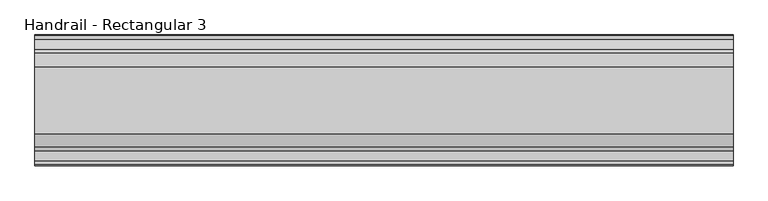
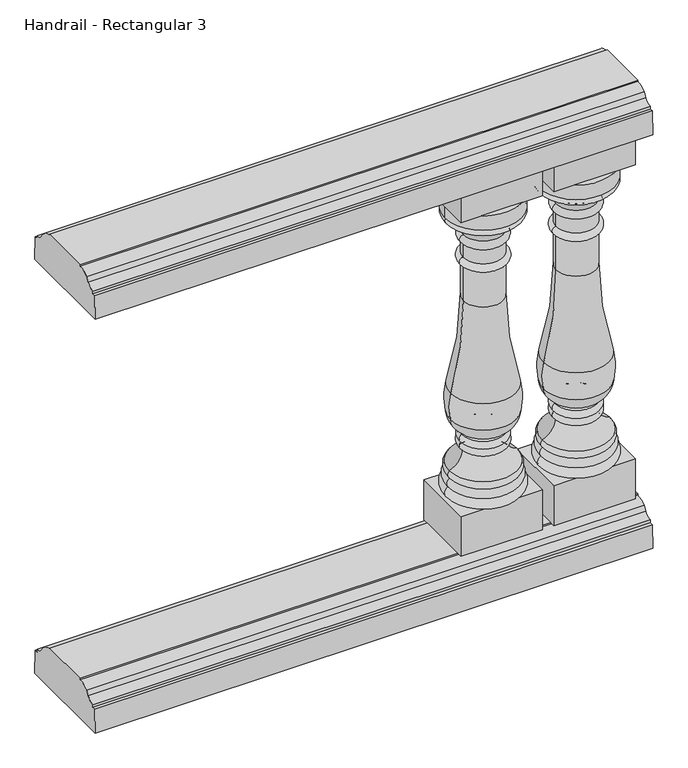
"""IFC4 building model written with IfcOpenShell, lengths in millimetres: railing geometry, Handrail - Rectangular 3."""

from ifc_helpers import new_model, si_unit, point, frame, frame_2d, origin, place, context, project, spatial, polyline, circle_curve, ellipse_curve, trimmed, segment, composite_curve, outline, extrude, source, transform, mapped, element, save
from ifc_brep_helpers import plane_surface, cylinder_surface, revolved_surface, advanced_brep


def handrail_rectangular_3_6dd137a3(model_context):
    return source(origin(), model_context, "Body", "SolidModel", [
        extrude(outline(composite_curve([segment(trimmed(circle_curve(frame_2d((-1771.1852268, 1054.89375)), 19.84375), [point((-1771.1852268, 1035.05))], [point((-1754.064785, 1044.8605607))], True, "CARTESIAN"), True, "CONTINUOUS"), segment(polyline([(-1754.064785, 1044.8605607), (-1747.604713, 1054.3201059)]), True, "CONTINUOUS"), segment(trimmed(circle_curve(frame_2d((-1723.5602268, 1027.90625)), 35.71875), [point((-1747.604713, 1054.3201059))], [point((-1723.5602268, 1063.625))], False, "CARTESIAN"), True, "CONTINUOUS"), segment(polyline([(-1723.5602268, 1063.625), (-1723.5602268, 1066.8), (-1607.6727268, 1066.8), (-1607.6727268, 1063.625)]), True, "CONTINUOUS"), segment(trimmed(circle_curve(frame_2d((-1607.6727268, 1027.90625)), 35.71875), [point((-1607.6727268, 1063.625))], [point((-1583.6282406, 1054.3201059))], False, "CARTESIAN"), True, "CONTINUOUS"), segment(polyline([(-1583.6282406, 1054.3201059), (-1577.1681686, 1044.8605607)]), True, "CONTINUOUS"), segment(trimmed(circle_curve(frame_2d((-1560.0477268, 1054.89375)), 19.84375), [point((-1577.1681686, 1044.8605607))], [point((-1560.0477268, 1035.05))], True, "CARTESIAN"), True, "CONTINUOUS"), segment(polyline([(-1560.0477268, 1035.05), (-1560.0477268, 1028.7), (-1552.9039768, 1028.7), (-1551.3164768, 974.725), (-1779.9164768, 974.725), (-1778.3289768, 1028.7), (-1771.1852268, 1028.7), (-1771.1852268, 1035.05)]), True, "CONTINUOUS")], self_intersect=False)), frame((11389.2521895, 0.0, 0.0), z_axis=(1.0, 0.0, 0.0), x_axis=(0.0, 1.0, 0.0)), (0.0, 0.0, 1.0), 1219.2),
        extrude(outline(composite_curve([segment(trimmed(circle_curve(frame_2d((-1771.1852268, 99.21875)), 19.84375), [point((-1771.1852268, 79.375))], [point((-1754.064785, 89.1855607))], True, "CARTESIAN"), True, "CONTINUOUS"), segment(polyline([(-1754.064785, 89.1855607), (-1747.604713, 98.6451059)]), True, "CONTINUOUS"), segment(trimmed(circle_curve(frame_2d((-1723.5602268, 72.23125)), 35.71875), [point((-1747.604713, 98.6451059))], [point((-1723.5602268, 107.95))], False, "CARTESIAN"), True, "CONTINUOUS"), segment(polyline([(-1723.5602268, 107.95), (-1723.5602268, 111.125), (-1607.6727268, 111.125), (-1607.6727268, 107.95)]), True, "CONTINUOUS"), segment(trimmed(circle_curve(frame_2d((-1607.6727268, 72.23125)), 35.71875), [point((-1607.6727268, 107.95))], [point((-1583.6282406, 98.6451059))], False, "CARTESIAN"), True, "CONTINUOUS"), segment(polyline([(-1583.6282406, 98.6451059), (-1577.1681686, 89.1855607)]), True, "CONTINUOUS"), segment(trimmed(circle_curve(frame_2d((-1560.0477268, 99.21875)), 19.84375), [point((-1577.1681686, 89.1855607))], [point((-1560.0477268, 79.375))], True, "CARTESIAN"), True, "CONTINUOUS"), segment(polyline([(-1560.0477268, 79.375), (-1560.0477268, 73.025), (-1552.9039768, 73.025), (-1551.3164768, 19.05), (-1779.9164768, 19.05), (-1778.3289768, 73.025), (-1771.1852268, 73.025), (-1771.1852268, 79.375)]), True, "CONTINUOUS")], self_intersect=False)), frame((11389.2521895, 0.0, 0.0), z_axis=(1.0, 0.0, 0.0), x_axis=(0.0, 1.0, 0.0)), (0.0, 0.0, 1.0), 1219.2),
        advanced_brep(
        [(12423.5084395, -1665.6164768, 849.3125), (12590.1959395, -1665.6164768, 849.3125), (12590.1959395, -1665.6164768, 882.65), (12423.5084395, -1665.6164768, 882.65), (12426.6834395, -1665.6164768, 849.3125), (12587.0209395, -1665.6164768, 849.3125), (12426.6834395, -1665.6164768, 835.025), (12587.0209395, -1665.6164768, 835.025), (12463.1959395, -1665.6164768, 796.925), (12550.5084395, -1665.6164768, 796.925), (12463.1959395, -1665.6164768, 777.875), (12550.5084395, -1665.6164768, 777.875), (12463.1959395, -1665.6164768, 744.5375), (12550.5084395, -1665.6164768, 744.5375), (12463.1959395, -1665.6164768, 727.075), (12550.5084395, -1665.6164768, 727.075), (12463.1959395, -1665.6164768, 644.525), (12550.5084395, -1665.6164768, 644.525), (12436.0074221, -1665.6164768, 440.2065586), (12577.696957, -1665.6164768, 440.2065586), (12434.8170661, -1665.6164768, 379.6643134), (12578.887313, -1665.6164768, 379.6643134), (12462.0281246, -1665.6164768, 340.8286685), (12551.6762545, -1665.6164768, 340.8286685), (12460.3028429, -1665.6164768, 336.3463085), (12553.4015362, -1665.6164768, 336.3463085), (12459.2271895, -1665.6164768, 319.0875), (12554.4771895, -1665.6164768, 319.0875), (12462.4021895, -1665.6164768, 301.625), (12551.3021895, -1665.6164768, 301.625), (12433.0334395, -1665.6164768, 261.9375), (12580.6709395, -1665.6164768, 261.9375), (12433.8271895, -1665.6164768, 244.475), (12579.8771895, -1665.6164768, 244.475), (12429.8584395, -1665.6164768, 225.425), (12583.8459395, -1665.6164768, 225.425), (12426.6834395, -1665.6164768, 203.2), (12587.0209395, -1665.6164768, 203.2), (12506.8521895, -1665.6164768, 203.2), (12506.8521895, -1665.6164768, 882.65)],
        [
            (0, 1, circle_curve(frame((12506.8521895, -1665.6164768, 849.3125), z_axis=(0.0, 0.0, 1.0), x_axis=(1.0, 0.0, 0.0)), 83.34375)),
            (1, 2),
            (2, 3, circle_curve(frame((12506.8521895, -1665.6164768, 882.65), z_axis=(0.0, 0.0, -1.0), x_axis=(1.0, 0.0, 0.0)), 83.34375)),
            (3, 0),
            (1, 0, circle_curve(frame((12506.8521895, -1665.6164768, 849.3125), z_axis=(0.0, 0.0, 1.0), x_axis=(1.0, 0.0, 0.0)), 83.34375)),
            (3, 2, circle_curve(frame((12506.8521895, -1665.6164768, 882.65), z_axis=(0.0, 0.0, -1.0), x_axis=(1.0, 0.0, 0.0)), 83.34375)),
            (4, 5, circle_curve(frame((12506.8521895, -1665.6164768, 849.3125), z_axis=(0.0, 0.0, 1.0), x_axis=(1.0, 0.0, 0.0)), 80.16875)),
            (5, 1),
            (0, 4),
            (5, 4, circle_curve(frame((12506.8521895, -1665.6164768, 849.3125), z_axis=(0.0, 0.0, 1.0), x_axis=(1.0, 0.0, 0.0)), 80.16875)),
            (6, 7, circle_curve(frame((12506.8521895, -1665.6164768, 835.025), z_axis=(0.0, 0.0, 1.0), x_axis=(1.0, 0.0, 0.0)), 80.16875)),
            (7, 5, circle_curve(frame((12580.5717208, -1665.6164768, 842.16875), z_axis=(0.0, -1.0, 0.0), x_axis=(1.0, 0.0, 0.0)), 9.6242187)),
            (4, 6, circle_curve(frame((12433.1326583, -1665.6164768, 842.16875), z_axis=(0.0, -1.0, 0.0), x_axis=(-1.0, 0.0, 0.0)), 9.6242187)),
            (7, 6, circle_curve(frame((12506.8521895, -1665.6164768, 835.025), z_axis=(0.0, 0.0, 1.0), x_axis=(1.0, 0.0, 0.0)), 80.16875)),
            (8, 9, circle_curve(frame((12506.8521895, -1665.6164768, 796.925), z_axis=(0.0, 0.0, 1.0), x_axis=(1.0, 0.0, 0.0)), 43.65625)),
            (9, 7, circle_curve(frame((12605.925244, -1665.6164768, 780.362802), z_axis=(0.0, 1.0, 0.0), x_axis=(1.0, 0.0, 0.0)), 57.8388159)),
            (6, 8, circle_curve(frame((12407.7791351, -1665.6164768, 780.362802), z_axis=(0.0, 1.0, 0.0), x_axis=(-1.0, 0.0, 0.0)), 57.8388159)),
            (9, 8, circle_curve(frame((12506.8521895, -1665.6164768, 796.925), z_axis=(0.0, 0.0, 1.0), x_axis=(1.0, 0.0, 0.0)), 43.65625)),
            (10, 11, circle_curve(frame((12506.8521895, -1665.6164768, 777.875), z_axis=(0.0, 0.0, 1.0), x_axis=(1.0, 0.0, 0.0)), 43.65625)),
            (11, 9, circle_curve(frame((12548.7621895, -1665.6164768, 787.4), z_axis=(0.0, -1.0, 0.0), x_axis=(1.0, 0.0, 0.0)), 9.68375)),
            (8, 10, circle_curve(frame((12464.9421895, -1665.6164768, 787.4), z_axis=(0.0, -1.0, 0.0), x_axis=(-1.0, 0.0, 0.0)), 9.68375)),
            (11, 10, circle_curve(frame((12506.8521895, -1665.6164768, 777.875), z_axis=(0.0, 0.0, 1.0), x_axis=(1.0, 0.0, 0.0)), 43.65625)),
            (12, 13, circle_curve(frame((12506.8521895, -1665.6164768, 744.5375), z_axis=(0.0, 0.0, 1.0), x_axis=(1.0, 0.0, 0.0)), 43.65625)),
            (13, 11),
            (10, 12),
            (13, 12, circle_curve(frame((12506.8521895, -1665.6164768, 744.5375), z_axis=(0.0, 0.0, 1.0), x_axis=(1.0, 0.0, 0.0)), 43.65625)),
            (14, 15, circle_curve(frame((12506.8521895, -1665.6164768, 727.075), z_axis=(0.0, 0.0, 1.0), x_axis=(1.0, 0.0, 0.0)), 43.65625)),
            (15, 13, circle_curve(frame((12550.5084395, -1665.6164768, 735.80625), z_axis=(0.0, -1.0, 0.0), x_axis=(1.0, 0.0, 0.0)), 8.73125)),
            (12, 14, circle_curve(frame((12463.1959395, -1665.6164768, 735.80625), z_axis=(0.0, -1.0, 0.0), x_axis=(-1.0, 0.0, 0.0)), 8.73125)),
            (15, 14, circle_curve(frame((12506.8521895, -1665.6164768, 727.075), z_axis=(0.0, 0.0, 1.0), x_axis=(1.0, 0.0, 0.0)), 43.65625)),
            (16, 17, circle_curve(frame((12506.8521895, -1665.6164768, 644.525), z_axis=(0.0, 0.0, 1.0), x_axis=(1.0, 0.0, 0.0)), 43.65625)),
            (17, 15),
            (14, 16),
            (17, 16, circle_curve(frame((12506.8521895, -1665.6164768, 644.525), z_axis=(0.0, 0.0, 1.0), x_axis=(1.0, 0.0, 0.0)), 43.65625)),
            (18, 19, circle_curve(frame((12506.8521895, -1665.6164768, 440.2065586), z_axis=(0.0, 0.0, 1.0), x_axis=(1.0, 0.0, 0.0)), 70.8447675)),
            (19, 17, circle_curve(frame((13285.2851891, -1665.6164768, 638.333048), z_axis=(0.0, 1.0, 0.0), x_axis=(1.0, 0.0, 0.0)), 734.8028389)),
            (16, 18, circle_curve(frame((11728.41919, -1665.6164768, 638.333048), z_axis=(0.0, 1.0, 0.0), x_axis=(-1.0, 0.0, 0.0)), 734.8028389)),
            (19, 18, circle_curve(frame((12506.8521895, -1665.6164768, 440.2065586), z_axis=(0.0, 0.0, 1.0), x_axis=(1.0, 0.0, 0.0)), 70.8447675)),
            (20, 21, circle_curve(frame((12506.8521895, -1665.6164768, 379.6643134), z_axis=(0.0, 0.0, 1.0), x_axis=(1.0, 0.0, 0.0)), 72.0351235)),
            (21, 19, circle_curve(frame((12419.7983349, -1665.6164768, 406.819198), z_axis=(0.0, -1.0, 0.0), x_axis=(1.0, 0.0, 0.0)), 161.3898718)),
            (18, 20, circle_curve(frame((12593.9060442, -1665.6164768, 406.819198), z_axis=(0.0, -1.0, 0.0), x_axis=(-1.0, 0.0, 0.0)), 161.3898718)),
            (21, 20, circle_curve(frame((12506.8521895, -1665.6164768, 379.6643134), z_axis=(0.0, 0.0, 1.0), x_axis=(1.0, 0.0, 0.0)), 72.0351235)),
            (22, 23, circle_curve(frame((12506.8521895, -1665.6164768, 340.8286685), z_axis=(0.0, 0.0, 1.0), x_axis=(1.0, 0.0, 0.0)), 44.8240649)),
            (23, 21, circle_curve(frame((12529.1572912, -1665.6164768, 385.5579203), z_axis=(0.0, -1.0, 0.0), x_axis=(1.0, 0.0, 0.0)), 50.0780358)),
            (20, 22, circle_curve(frame((12484.5470879, -1665.6164768, 385.5579203), z_axis=(0.0, -1.0, 0.0), x_axis=(-1.0, 0.0, 0.0)), 50.0780358)),
            (23, 22, circle_curve(frame((12506.8521895, -1665.6164768, 340.8286685), z_axis=(0.0, 0.0, 1.0), x_axis=(1.0, 0.0, 0.0)), 44.8240649)),
            (24, 25, circle_curve(frame((12506.8521895, -1665.6164768, 336.3463085), z_axis=(0.0, 0.0, 1.0), x_axis=(1.0, 0.0, 0.0)), 46.5493467)),
            (25, 23, circle_curve(frame((12554.4771895, -1665.6164768, 339.3335472), z_axis=(0.0, 1.0, 0.0), x_axis=(1.0, 0.0, 0.0)), 3.175)),
            (22, 24, circle_curve(frame((12459.2271895, -1665.6164768, 339.3335472), z_axis=(0.0, 1.0, 0.0), x_axis=(-1.0, 0.0, 0.0)), 3.175)),
            (25, 24, circle_curve(frame((12506.8521895, -1665.6164768, 336.3463085), z_axis=(0.0, 0.0, 1.0), x_axis=(1.0, 0.0, 0.0)), 46.5493467)),
            (26, 27, circle_curve(frame((12506.8521895, -1665.6164768, 319.0875), z_axis=(0.0, 0.0, 1.0), x_axis=(1.0, 0.0, 0.0)), 47.625)),
            (27, 25, circle_curve(frame((12549.4008248, -1665.6164768, 327.4340404), z_axis=(0.0, -1.0, 0.0), x_axis=(1.0, 0.0, 0.0)), 9.7690437)),
            (24, 26, circle_curve(frame((12464.3035543, -1665.6164768, 327.4340404), z_axis=(0.0, -1.0, 0.0), x_axis=(-1.0, 0.0, 0.0)), 9.7690437)),
            (27, 26, circle_curve(frame((12506.8521895, -1665.6164768, 319.0875), z_axis=(0.0, 0.0, 1.0), x_axis=(1.0, 0.0, 0.0)), 47.625)),
            (28, 29, circle_curve(frame((12506.8521895, -1665.6164768, 301.625), z_axis=(0.0, 0.0, 1.0), x_axis=(1.0, 0.0, 0.0)), 44.45)),
            (29, 27, circle_curve(frame((12549.8635177, -1665.6164768, 310.9064631), z_axis=(0.0, -1.0, 0.0), x_axis=(1.0, 0.0, 0.0)), 9.3923018)),
            (26, 28, circle_curve(frame((12463.8408614, -1665.6164768, 310.9064631), z_axis=(0.0, -1.0, 0.0), x_axis=(-1.0, 0.0, 0.0)), 9.3923018)),
            (29, 28, circle_curve(frame((12506.8521895, -1665.6164768, 301.625), z_axis=(0.0, 0.0, 1.0), x_axis=(1.0, 0.0, 0.0)), 44.45)),
            (30, 31, circle_curve(frame((12506.8521895, -1665.6164768, 261.9375), z_axis=(0.0, 0.0, 1.0), x_axis=(1.0, 0.0, 0.0)), 73.81875)),
            (31, 29, circle_curve(frame((12592.8024429, -1665.6164768, 301.625), z_axis=(0.0, 1.0, 0.0), x_axis=(1.0, 0.0, 0.0)), 41.5002534)),
            (28, 30, circle_curve(frame((12420.9019362, -1665.6164768, 301.625), z_axis=(0.0, 1.0, 0.0), x_axis=(-1.0, 0.0, 0.0)), 41.5002534)),
            (31, 30, circle_curve(frame((12506.8521895, -1665.6164768, 261.9375), z_axis=(0.0, 0.0, 1.0), x_axis=(1.0, 0.0, 0.0)), 73.81875)),
            (32, 33, circle_curve(frame((12506.8521895, -1665.6164768, 244.475), z_axis=(0.0, 0.0, 1.0), x_axis=(1.0, 0.0, 0.0)), 73.025)),
            (33, 31, circle_curve(frame((12571.3664257, -1665.6164768, 253.6111427), z_axis=(0.0, -1.0, 0.0), x_axis=(1.0, 0.0, 0.0)), 12.4860804)),
            (30, 32, circle_curve(frame((12442.3379534, -1665.6164768, 253.6111427), z_axis=(0.0, -1.0, 0.0), x_axis=(-1.0, 0.0, 0.0)), 12.4860804)),
            (33, 32, circle_curve(frame((12506.8521895, -1665.6164768, 244.475), z_axis=(0.0, 0.0, 1.0), x_axis=(1.0, 0.0, 0.0)), 73.025)),
            (34, 35, circle_curve(frame((12506.8521895, -1665.6164768, 225.425), z_axis=(0.0, 0.0, 1.0), x_axis=(1.0, 0.0, 0.0)), 76.99375)),
            (35, 33, circle_curve(frame((12573.2024736, -1665.6164768, 233.1460227), z_axis=(0.0, -1.0, 0.0), x_axis=(1.0, 0.0, 0.0)), 13.1490516)),
            (32, 34, circle_curve(frame((12440.5019054, -1665.6164768, 233.1460227), z_axis=(0.0, -1.0, 0.0), x_axis=(-1.0, 0.0, 0.0)), 13.1490516)),
            (35, 34, circle_curve(frame((12506.8521895, -1665.6164768, 225.425), z_axis=(0.0, 0.0, 1.0), x_axis=(1.0, 0.0, 0.0)), 76.99375)),
            (36, 37, circle_curve(frame((12506.8521895, -1665.6164768, 203.2), z_axis=(0.0, 0.0, 1.0), x_axis=(1.0, 0.0, 0.0)), 80.16875)),
            (37, 35, circle_curve(frame((12576.8722788, -1665.6164768, 213.089477), z_axis=(0.0, -1.0, 0.0), x_axis=(1.0, 0.0, 0.0)), 14.1702883)),
            (34, 36, circle_curve(frame((12436.8321003, -1665.6164768, 213.089477), z_axis=(0.0, -1.0, 0.0), x_axis=(-1.0, 0.0, 0.0)), 14.1702883)),
            (37, 36, circle_curve(frame((12506.8521895, -1665.6164768, 203.2), z_axis=(0.0, 0.0, 1.0), x_axis=(1.0, 0.0, 0.0)), 80.16875)),
            (38, 37),
            (36, 38),
            (2, 39),
            (39, 3),
        ],
        [
            cylinder_surface(frame((12506.8521895, -1665.6164768, 831.85), z_axis=(0.0, 0.0, -1.0), x_axis=(1.0, 0.0, 0.0)), 83.34375),
            plane_surface(frame((12506.8521895, -1665.6164768, 849.3125), z_axis=(0.0, 0.0, -1.0), x_axis=(1.0, 0.0, 0.0))),
            revolved_surface(trimmed(ellipse_curve(frame((12580.5717208, -1665.6164768, 842.16875), z_axis=(0.0, 1.0, 0.0), x_axis=(1.0, 0.0, 0.0)), 9.6242187, 9.6242187), [point((12587.0209395, -1665.6164768, 849.3125))], [point((12587.0209395, -1665.6164768, 835.025))], True, "CARTESIAN"), (12506.8521895, -1665.6164768, 831.85), (0.0, 0.0, -1.0)),
            revolved_surface(trimmed(ellipse_curve(frame((12605.925244, -1665.6164768, 780.362802), z_axis=(0.0, -1.0, 0.0), x_axis=(1.0, 0.0, 0.0)), 57.8388159, 57.8388159), [point((12587.0209395, -1665.6164768, 835.025))], [point((12550.5084395, -1665.6164768, 796.925))], True, "CARTESIAN"), (12506.8521895, -1665.6164768, 831.85), (0.0, 0.0, -1.0)),
            revolved_surface(trimmed(ellipse_curve(frame((12548.7621895, -1665.6164768, 787.4), z_axis=(0.0, 1.0, 0.0), x_axis=(1.0, 0.0, 0.0)), 9.68375, 9.68375), [point((12550.5084395, -1665.6164768, 796.925))], [point((12550.5084395, -1665.6164768, 777.875))], True, "CARTESIAN"), (12506.8521895, -1665.6164768, 831.85), (0.0, 0.0, -1.0)),
            cylinder_surface(frame((12506.8521895, -1665.6164768, 831.85), z_axis=(0.0, 0.0, -1.0), x_axis=(1.0, 0.0, 0.0)), 43.65625),
            revolved_surface(trimmed(ellipse_curve(frame((12550.5084395, -1665.6164768, 735.80625), z_axis=(0.0, 1.0, 0.0), x_axis=(1.0, 0.0, 0.0)), 8.73125, 8.73125), [point((12550.5084395, -1665.6164768, 744.5375))], [point((12550.5084395, -1665.6164768, 727.075))], True, "CARTESIAN"), (12506.8521895, -1665.6164768, 831.85), (0.0, 0.0, -1.0)),
            revolved_surface(trimmed(ellipse_curve(frame((13285.2851891, -1665.6164768, 638.333048), z_axis=(0.0, -1.0, 0.0), x_axis=(1.0, 0.0, 0.0)), 734.8028389, 734.8028389), [point((12550.5084395, -1665.6164768, 644.525))], [point((12577.696957, -1665.6164768, 440.2065586))], True, "CARTESIAN"), (12506.8521895, -1665.6164768, 831.85), (0.0, 0.0, -1.0)),
            revolved_surface(trimmed(ellipse_curve(frame((12419.7983349, -1665.6164768, 406.819198), z_axis=(0.0, 1.0, 0.0), x_axis=(1.0, 0.0, 0.0)), 161.3898718, 161.3898718), [point((12577.696957, -1665.6164768, 440.2065586))], [point((12578.887313, -1665.6164768, 379.6643134))], True, "CARTESIAN"), (12506.8521895, -1665.6164768, 831.85), (0.0, 0.0, -1.0)),
            revolved_surface(trimmed(ellipse_curve(frame((12529.1572912, -1665.6164768, 385.5579203), z_axis=(0.0, 1.0, 0.0), x_axis=(1.0, 0.0, 0.0)), 50.0780358, 50.0780358), [point((12578.887313, -1665.6164768, 379.6643134))], [point((12551.6762545, -1665.6164768, 340.8286685))], True, "CARTESIAN"), (12506.8521895, -1665.6164768, 831.85), (0.0, 0.0, -1.0)),
            revolved_surface(trimmed(ellipse_curve(frame((12554.4771895, -1665.6164768, 339.3335472), z_axis=(0.0, -1.0, 0.0), x_axis=(1.0, 0.0, 0.0)), 3.175, 3.175), [point((12551.6762545, -1665.6164768, 340.8286685))], [point((12553.4015362, -1665.6164768, 336.3463085))], True, "CARTESIAN"), (12506.8521895, -1665.6164768, 831.85), (0.0, 0.0, -1.0)),
            revolved_surface(trimmed(ellipse_curve(frame((12549.4008248, -1665.6164768, 327.4340404), z_axis=(0.0, 1.0, 0.0), x_axis=(1.0, 0.0, 0.0)), 9.7690437, 9.7690437), [point((12553.4015362, -1665.6164768, 336.3463085))], [point((12554.4771895, -1665.6164768, 319.0875))], True, "CARTESIAN"), (12506.8521895, -1665.6164768, 831.85), (0.0, 0.0, -1.0)),
            revolved_surface(trimmed(ellipse_curve(frame((12549.8635177, -1665.6164768, 310.9064631), z_axis=(0.0, 1.0, 0.0), x_axis=(1.0, 0.0, 0.0)), 9.3923018, 9.3923018), [point((12554.4771895, -1665.6164768, 319.0875))], [point((12551.3021895, -1665.6164768, 301.625))], True, "CARTESIAN"), (12506.8521895, -1665.6164768, 831.85), (0.0, 0.0, -1.0)),
            revolved_surface(trimmed(ellipse_curve(frame((12592.8024429, -1665.6164768, 301.625), z_axis=(0.0, -1.0, 0.0), x_axis=(1.0, 0.0, 0.0)), 41.5002534, 41.5002534), [point((12551.3021895, -1665.6164768, 301.625))], [point((12580.6709395, -1665.6164768, 261.9375))], True, "CARTESIAN"), (12506.8521895, -1665.6164768, 831.85), (0.0, 0.0, -1.0)),
            revolved_surface(trimmed(ellipse_curve(frame((12571.3664257, -1665.6164768, 253.6111427), z_axis=(0.0, 1.0, 0.0), x_axis=(1.0, 0.0, 0.0)), 12.4860804, 12.4860804), [point((12580.6709395, -1665.6164768, 261.9375))], [point((12579.8771895, -1665.6164768, 244.475))], True, "CARTESIAN"), (12506.8521895, -1665.6164768, 831.85), (0.0, 0.0, -1.0)),
            revolved_surface(trimmed(ellipse_curve(frame((12573.2024736, -1665.6164768, 233.1460227), z_axis=(0.0, 1.0, 0.0), x_axis=(1.0, 0.0, 0.0)), 13.1490516, 13.1490516), [point((12579.8771895, -1665.6164768, 244.475))], [point((12583.8459395, -1665.6164768, 225.425))], True, "CARTESIAN"), (12506.8521895, -1665.6164768, 831.85), (0.0, 0.0, -1.0)),
            revolved_surface(trimmed(ellipse_curve(frame((12576.8722788, -1665.6164768, 213.089477), z_axis=(0.0, 1.0, 0.0), x_axis=(1.0, 0.0, 0.0)), 14.1702883, 14.1702883), [point((12583.8459395, -1665.6164768, 225.425))], [point((12587.0209395, -1665.6164768, 203.2))], True, "CARTESIAN"), (12506.8521895, -1665.6164768, 831.85), (0.0, 0.0, -1.0)),
            plane_surface(frame((12506.8521895, -1665.6164768, 203.2), z_axis=(0.0, 0.0, -1.0), x_axis=(1.0, 0.0, 0.0))),
            plane_surface(frame((12506.8521895, -1665.6164768, 882.65), z_axis=(0.0, 0.0, 1.0), x_axis=(1.0, 0.0, 0.0))),
        ],
        [
            (0, [[1, 2, 3, 4]]),
            (0, [[5, -4, 6, -2]]),
            (1, [[7, 8, -1, 9]]),
            (1, [[10, -9, -5, -8]]),
            (2, [[11, 12, -7, 13]]),
            (2, [[14, -13, -10, -12]]),
            (3, [[15, 16, -11, 17]]),
            (3, [[18, -17, -14, -16]]),
            (4, [[19, 20, -15, 21]]),
            (4, [[22, -21, -18, -20]]),
            (5, [[23, 24, -19, 25]]),
            (5, [[26, -25, -22, -24]]),
            (6, [[27, 28, -23, 29]]),
            (6, [[30, -29, -26, -28]]),
            (5, [[31, 32, -27, 33]]),
            (5, [[34, -33, -30, -32]]),
            (7, [[35, 36, -31, 37]]),
            (7, [[38, -37, -34, -36]]),
            (8, [[39, 40, -35, 41]]),
            (8, [[42, -41, -38, -40]]),
            (9, [[43, 44, -39, 45]]),
            (9, [[46, -45, -42, -44]]),
            (10, [[47, 48, -43, 49]]),
            (10, [[50, -49, -46, -48]]),
            (11, [[51, 52, -47, 53]]),
            (11, [[54, -53, -50, -52]]),
            (12, [[55, 56, -51, 57]]),
            (12, [[58, -57, -54, -56]]),
            (13, [[59, 60, -55, 61]]),
            (13, [[62, -61, -58, -60]]),
            (14, [[63, 64, -59, 65]]),
            (14, [[66, -65, -62, -64]]),
            (15, [[67, 68, -63, 69]]),
            (15, [[70, -69, -66, -68]]),
            (16, [[71, 72, -67, 73]]),
            (16, [[74, -73, -70, -72]]),
            (17, [[75, -71, 76]]),
            (17, [[-76, -74, -75]]),
            (18, [[-3, 77, 78]]),
            (18, [[-6, -78, -77]]),
        ],
    ),
        extrude(outline(polyline([(12417.9521895, -1735.4664768), (12417.9521895, -1595.7664768), (12595.7521895, -1595.7664768), (12595.7521895, -1735.4664768), (12417.9521895, -1735.4664768)])), frame((0.0, 0.0, 111.125), z_axis=(0.0, 0.0, 1.0), x_axis=(1.0, 0.0, 0.0)), (0.0, 0.0, 1.0), 92.075),
        extrude(outline(polyline([(12417.9521895, -1595.7664768), (12595.7521895, -1595.7664768), (12595.7521895, -1735.4664768), (12417.9521895, -1735.4664768), (12417.9521895, -1595.7664768)])), frame((0.0, 0.0, 882.65), z_axis=(0.0, 0.0, 1.0), x_axis=(1.0, 0.0, 0.0)), (0.0, 0.0, 1.0), 92.075),
        advanced_brep(
        [(12220.3084395, -1665.6164768, 849.3125), (12386.9959395, -1665.6164768, 849.3125), (12386.9959395, -1665.6164768, 882.65), (12220.3084395, -1665.6164768, 882.65), (12223.4834395, -1665.6164768, 849.3125), (12383.8209395, -1665.6164768, 849.3125), (12223.4834395, -1665.6164768, 835.025), (12383.8209395, -1665.6164768, 835.025), (12259.9959395, -1665.6164768, 796.925), (12347.3084395, -1665.6164768, 796.925), (12259.9959395, -1665.6164768, 777.875), (12347.3084395, -1665.6164768, 777.875), (12259.9959395, -1665.6164768, 744.5375), (12347.3084395, -1665.6164768, 744.5375), (12259.9959395, -1665.6164768, 727.075), (12347.3084395, -1665.6164768, 727.075), (12259.9959395, -1665.6164768, 644.525), (12347.3084395, -1665.6164768, 644.525), (12232.8074221, -1665.6164768, 440.2065586), (12374.496957, -1665.6164768, 440.2065586), (12231.6170661, -1665.6164768, 379.6643134), (12375.687313, -1665.6164768, 379.6643134), (12258.8281246, -1665.6164768, 340.8286685), (12348.4762545, -1665.6164768, 340.8286685), (12257.1028429, -1665.6164768, 336.3463085), (12350.2015362, -1665.6164768, 336.3463085), (12256.0271895, -1665.6164768, 319.0875), (12351.2771895, -1665.6164768, 319.0875), (12259.2021895, -1665.6164768, 301.625), (12348.1021895, -1665.6164768, 301.625), (12229.8334395, -1665.6164768, 261.9375), (12377.4709395, -1665.6164768, 261.9375), (12230.6271895, -1665.6164768, 244.475), (12376.6771895, -1665.6164768, 244.475), (12226.6584395, -1665.6164768, 225.425), (12380.6459395, -1665.6164768, 225.425), (12223.4834395, -1665.6164768, 203.2), (12383.8209395, -1665.6164768, 203.2), (12303.6521895, -1665.6164768, 203.2), (12303.6521895, -1665.6164768, 882.65)],
        [
            (0, 1, circle_curve(frame((12303.6521895, -1665.6164768, 849.3125), z_axis=(0.0, 0.0, 1.0), x_axis=(1.0, 0.0, 0.0)), 83.34375)),
            (1, 2),
            (2, 3, circle_curve(frame((12303.6521895, -1665.6164768, 882.65), z_axis=(0.0, 0.0, -1.0), x_axis=(1.0, 0.0, 0.0)), 83.34375)),
            (3, 0),
            (1, 0, circle_curve(frame((12303.6521895, -1665.6164768, 849.3125), z_axis=(0.0, 0.0, 1.0), x_axis=(1.0, 0.0, 0.0)), 83.34375)),
            (3, 2, circle_curve(frame((12303.6521895, -1665.6164768, 882.65), z_axis=(0.0, 0.0, -1.0), x_axis=(1.0, 0.0, 0.0)), 83.34375)),
            (4, 5, circle_curve(frame((12303.6521895, -1665.6164768, 849.3125), z_axis=(0.0, 0.0, 1.0), x_axis=(1.0, 0.0, 0.0)), 80.16875)),
            (5, 1),
            (0, 4),
            (5, 4, circle_curve(frame((12303.6521895, -1665.6164768, 849.3125), z_axis=(0.0, 0.0, 1.0), x_axis=(1.0, 0.0, 0.0)), 80.16875)),
            (6, 7, circle_curve(frame((12303.6521895, -1665.6164768, 835.025), z_axis=(0.0, 0.0, 1.0), x_axis=(1.0, 0.0, 0.0)), 80.16875)),
            (7, 5, circle_curve(frame((12377.3717208, -1665.6164768, 842.16875), z_axis=(0.0, -1.0, 0.0), x_axis=(1.0, 0.0, 0.0)), 9.6242187)),
            (4, 6, circle_curve(frame((12229.9326583, -1665.6164768, 842.16875), z_axis=(0.0, -1.0, 0.0), x_axis=(-1.0, 0.0, 0.0)), 9.6242187)),
            (7, 6, circle_curve(frame((12303.6521895, -1665.6164768, 835.025), z_axis=(0.0, 0.0, 1.0), x_axis=(1.0, 0.0, 0.0)), 80.16875)),
            (8, 9, circle_curve(frame((12303.6521895, -1665.6164768, 796.925), z_axis=(0.0, 0.0, 1.0), x_axis=(1.0, 0.0, 0.0)), 43.65625)),
            (9, 7, circle_curve(frame((12402.725244, -1665.6164768, 780.362802), z_axis=(0.0, 1.0, 0.0), x_axis=(1.0, 0.0, 0.0)), 57.8388159)),
            (6, 8, circle_curve(frame((12204.5791351, -1665.6164768, 780.362802), z_axis=(0.0, 1.0, 0.0), x_axis=(-1.0, 0.0, 0.0)), 57.8388159)),
            (9, 8, circle_curve(frame((12303.6521895, -1665.6164768, 796.925), z_axis=(0.0, 0.0, 1.0), x_axis=(1.0, 0.0, 0.0)), 43.65625)),
            (10, 11, circle_curve(frame((12303.6521895, -1665.6164768, 777.875), z_axis=(0.0, 0.0, 1.0), x_axis=(1.0, 0.0, 0.0)), 43.65625)),
            (11, 9, circle_curve(frame((12345.5621895, -1665.6164768, 787.4), z_axis=(0.0, -1.0, 0.0), x_axis=(1.0, 0.0, 0.0)), 9.68375)),
            (8, 10, circle_curve(frame((12261.7421895, -1665.6164768, 787.4), z_axis=(0.0, -1.0, 0.0), x_axis=(-1.0, 0.0, 0.0)), 9.68375)),
            (11, 10, circle_curve(frame((12303.6521895, -1665.6164768, 777.875), z_axis=(0.0, 0.0, 1.0), x_axis=(1.0, 0.0, 0.0)), 43.65625)),
            (12, 13, circle_curve(frame((12303.6521895, -1665.6164768, 744.5375), z_axis=(0.0, 0.0, 1.0), x_axis=(1.0, 0.0, 0.0)), 43.65625)),
            (13, 11),
            (10, 12),
            (13, 12, circle_curve(frame((12303.6521895, -1665.6164768, 744.5375), z_axis=(0.0, 0.0, 1.0), x_axis=(1.0, 0.0, 0.0)), 43.65625)),
            (14, 15, circle_curve(frame((12303.6521895, -1665.6164768, 727.075), z_axis=(0.0, 0.0, 1.0), x_axis=(1.0, 0.0, 0.0)), 43.65625)),
            (15, 13, circle_curve(frame((12347.3084395, -1665.6164768, 735.80625), z_axis=(0.0, -1.0, 0.0), x_axis=(1.0, 0.0, 0.0)), 8.73125)),
            (12, 14, circle_curve(frame((12259.9959395, -1665.6164768, 735.80625), z_axis=(0.0, -1.0, 0.0), x_axis=(-1.0, 0.0, 0.0)), 8.73125)),
            (15, 14, circle_curve(frame((12303.6521895, -1665.6164768, 727.075), z_axis=(0.0, 0.0, 1.0), x_axis=(1.0, 0.0, 0.0)), 43.65625)),
            (16, 17, circle_curve(frame((12303.6521895, -1665.6164768, 644.525), z_axis=(0.0, 0.0, 1.0), x_axis=(1.0, 0.0, 0.0)), 43.65625)),
            (17, 15),
            (14, 16),
            (17, 16, circle_curve(frame((12303.6521895, -1665.6164768, 644.525), z_axis=(0.0, 0.0, 1.0), x_axis=(1.0, 0.0, 0.0)), 43.65625)),
            (18, 19, circle_curve(frame((12303.6521895, -1665.6164768, 440.2065586), z_axis=(0.0, 0.0, 1.0), x_axis=(1.0, 0.0, 0.0)), 70.8447675)),
            (19, 17, circle_curve(frame((13082.0851891, -1665.6164768, 638.333048), z_axis=(0.0, 1.0, 0.0), x_axis=(1.0, 0.0, 0.0)), 734.8028389)),
            (16, 18, circle_curve(frame((11525.21919, -1665.6164768, 638.333048), z_axis=(0.0, 1.0, 0.0), x_axis=(-1.0, 0.0, 0.0)), 734.8028389)),
            (19, 18, circle_curve(frame((12303.6521895, -1665.6164768, 440.2065586), z_axis=(0.0, 0.0, 1.0), x_axis=(1.0, 0.0, 0.0)), 70.8447675)),
            (20, 21, circle_curve(frame((12303.6521895, -1665.6164768, 379.6643134), z_axis=(0.0, 0.0, 1.0), x_axis=(1.0, 0.0, 0.0)), 72.0351235)),
            (21, 19, circle_curve(frame((12216.5983349, -1665.6164768, 406.819198), z_axis=(0.0, -1.0, 0.0), x_axis=(1.0, 0.0, 0.0)), 161.3898718)),
            (18, 20, circle_curve(frame((12390.7060442, -1665.6164768, 406.819198), z_axis=(0.0, -1.0, 0.0), x_axis=(-1.0, 0.0, 0.0)), 161.3898718)),
            (21, 20, circle_curve(frame((12303.6521895, -1665.6164768, 379.6643134), z_axis=(0.0, 0.0, 1.0), x_axis=(1.0, 0.0, 0.0)), 72.0351235)),
            (22, 23, circle_curve(frame((12303.6521895, -1665.6164768, 340.8286685), z_axis=(0.0, 0.0, 1.0), x_axis=(1.0, 0.0, 0.0)), 44.8240649)),
            (23, 21, circle_curve(frame((12325.9572912, -1665.6164768, 385.5579203), z_axis=(0.0, -1.0, 0.0), x_axis=(1.0, 0.0, 0.0)), 50.0780358)),
            (20, 22, circle_curve(frame((12281.3470879, -1665.6164768, 385.5579203), z_axis=(0.0, -1.0, 0.0), x_axis=(-1.0, 0.0, 0.0)), 50.0780358)),
            (23, 22, circle_curve(frame((12303.6521895, -1665.6164768, 340.8286685), z_axis=(0.0, 0.0, 1.0), x_axis=(1.0, 0.0, 0.0)), 44.8240649)),
            (24, 25, circle_curve(frame((12303.6521895, -1665.6164768, 336.3463085), z_axis=(0.0, 0.0, 1.0), x_axis=(1.0, 0.0, 0.0)), 46.5493467)),
            (25, 23, circle_curve(frame((12351.2771895, -1665.6164768, 339.3335472), z_axis=(0.0, 1.0, 0.0), x_axis=(1.0, 0.0, 0.0)), 3.175)),
            (22, 24, circle_curve(frame((12256.0271895, -1665.6164768, 339.3335472), z_axis=(0.0, 1.0, 0.0), x_axis=(-1.0, 0.0, 0.0)), 3.175)),
            (25, 24, circle_curve(frame((12303.6521895, -1665.6164768, 336.3463085), z_axis=(0.0, 0.0, 1.0), x_axis=(1.0, 0.0, 0.0)), 46.5493467)),
            (26, 27, circle_curve(frame((12303.6521895, -1665.6164768, 319.0875), z_axis=(0.0, 0.0, 1.0), x_axis=(1.0, 0.0, 0.0)), 47.625)),
            (27, 25, circle_curve(frame((12346.2008248, -1665.6164768, 327.4340404), z_axis=(0.0, -1.0, 0.0), x_axis=(1.0, 0.0, 0.0)), 9.7690437)),
            (24, 26, circle_curve(frame((12261.1035543, -1665.6164768, 327.4340404), z_axis=(0.0, -1.0, 0.0), x_axis=(-1.0, 0.0, 0.0)), 9.7690437)),
            (27, 26, circle_curve(frame((12303.6521895, -1665.6164768, 319.0875), z_axis=(0.0, 0.0, 1.0), x_axis=(1.0, 0.0, 0.0)), 47.625)),
            (28, 29, circle_curve(frame((12303.6521895, -1665.6164768, 301.625), z_axis=(0.0, 0.0, 1.0), x_axis=(1.0, 0.0, 0.0)), 44.45)),
            (29, 27, circle_curve(frame((12346.6635177, -1665.6164768, 310.9064631), z_axis=(0.0, -1.0, 0.0), x_axis=(1.0, 0.0, 0.0)), 9.3923018)),
            (26, 28, circle_curve(frame((12260.6408614, -1665.6164768, 310.9064631), z_axis=(0.0, -1.0, 0.0), x_axis=(-1.0, 0.0, 0.0)), 9.3923018)),
            (29, 28, circle_curve(frame((12303.6521895, -1665.6164768, 301.625), z_axis=(0.0, 0.0, 1.0), x_axis=(1.0, 0.0, 0.0)), 44.45)),
            (30, 31, circle_curve(frame((12303.6521895, -1665.6164768, 261.9375), z_axis=(0.0, 0.0, 1.0), x_axis=(1.0, 0.0, 0.0)), 73.81875)),
            (31, 29, circle_curve(frame((12389.6024429, -1665.6164768, 301.625), z_axis=(0.0, 1.0, 0.0), x_axis=(1.0, 0.0, 0.0)), 41.5002534)),
            (28, 30, circle_curve(frame((12217.7019362, -1665.6164768, 301.625), z_axis=(0.0, 1.0, 0.0), x_axis=(-1.0, 0.0, 0.0)), 41.5002534)),
            (31, 30, circle_curve(frame((12303.6521895, -1665.6164768, 261.9375), z_axis=(0.0, 0.0, 1.0), x_axis=(1.0, 0.0, 0.0)), 73.81875)),
            (32, 33, circle_curve(frame((12303.6521895, -1665.6164768, 244.475), z_axis=(0.0, 0.0, 1.0), x_axis=(1.0, 0.0, 0.0)), 73.025)),
            (33, 31, circle_curve(frame((12368.1664257, -1665.6164768, 253.6111427), z_axis=(0.0, -1.0, 0.0), x_axis=(1.0, 0.0, 0.0)), 12.4860804)),
            (30, 32, circle_curve(frame((12239.1379534, -1665.6164768, 253.6111427), z_axis=(0.0, -1.0, 0.0), x_axis=(-1.0, 0.0, 0.0)), 12.4860804)),
            (33, 32, circle_curve(frame((12303.6521895, -1665.6164768, 244.475), z_axis=(0.0, 0.0, 1.0), x_axis=(1.0, 0.0, 0.0)), 73.025)),
            (34, 35, circle_curve(frame((12303.6521895, -1665.6164768, 225.425), z_axis=(0.0, 0.0, 1.0), x_axis=(1.0, 0.0, 0.0)), 76.99375)),
            (35, 33, circle_curve(frame((12370.0024736, -1665.6164768, 233.1460227), z_axis=(0.0, -1.0, 0.0), x_axis=(1.0, 0.0, 0.0)), 13.1490516)),
            (32, 34, circle_curve(frame((12237.3019054, -1665.6164768, 233.1460227), z_axis=(0.0, -1.0, 0.0), x_axis=(-1.0, 0.0, 0.0)), 13.1490516)),
            (35, 34, circle_curve(frame((12303.6521895, -1665.6164768, 225.425), z_axis=(0.0, 0.0, 1.0), x_axis=(1.0, 0.0, 0.0)), 76.99375)),
            (36, 37, circle_curve(frame((12303.6521895, -1665.6164768, 203.2), z_axis=(0.0, 0.0, 1.0), x_axis=(1.0, 0.0, 0.0)), 80.16875)),
            (37, 35, circle_curve(frame((12373.6722788, -1665.6164768, 213.089477), z_axis=(0.0, -1.0, 0.0), x_axis=(1.0, 0.0, 0.0)), 14.1702883)),
            (34, 36, circle_curve(frame((12233.6321003, -1665.6164768, 213.089477), z_axis=(0.0, -1.0, 0.0), x_axis=(-1.0, 0.0, 0.0)), 14.1702883)),
            (37, 36, circle_curve(frame((12303.6521895, -1665.6164768, 203.2), z_axis=(0.0, 0.0, 1.0), x_axis=(1.0, 0.0, 0.0)), 80.16875)),
            (38, 37),
            (36, 38),
            (2, 39),
            (39, 3),
        ],
        [
            cylinder_surface(frame((12303.6521895, -1665.6164768, 831.85), z_axis=(0.0, 0.0, -1.0), x_axis=(1.0, 0.0, 0.0)), 83.34375),
            plane_surface(frame((12303.6521895, -1665.6164768, 849.3125), z_axis=(0.0, 0.0, -1.0), x_axis=(1.0, 0.0, 0.0))),
            revolved_surface(trimmed(ellipse_curve(frame((12377.3717208, -1665.6164768, 842.16875), z_axis=(0.0, 1.0, 0.0), x_axis=(1.0, 0.0, 0.0)), 9.6242187, 9.6242187), [point((12383.8209395, -1665.6164768, 849.3125))], [point((12383.8209395, -1665.6164768, 835.025))], True, "CARTESIAN"), (12303.6521895, -1665.6164768, 831.85), (0.0, 0.0, -1.0)),
            revolved_surface(trimmed(ellipse_curve(frame((12402.725244, -1665.6164768, 780.362802), z_axis=(0.0, -1.0, 0.0), x_axis=(1.0, 0.0, 0.0)), 57.8388159, 57.8388159), [point((12383.8209395, -1665.6164768, 835.025))], [point((12347.3084395, -1665.6164768, 796.925))], True, "CARTESIAN"), (12303.6521895, -1665.6164768, 831.85), (0.0, 0.0, -1.0)),
            revolved_surface(trimmed(ellipse_curve(frame((12345.5621895, -1665.6164768, 787.4), z_axis=(0.0, 1.0, 0.0), x_axis=(1.0, 0.0, 0.0)), 9.68375, 9.68375), [point((12347.3084395, -1665.6164768, 796.925))], [point((12347.3084395, -1665.6164768, 777.875))], True, "CARTESIAN"), (12303.6521895, -1665.6164768, 831.85), (0.0, 0.0, -1.0)),
            cylinder_surface(frame((12303.6521895, -1665.6164768, 831.85), z_axis=(0.0, 0.0, -1.0), x_axis=(1.0, 0.0, 0.0)), 43.65625),
            revolved_surface(trimmed(ellipse_curve(frame((12347.3084395, -1665.6164768, 735.80625), z_axis=(0.0, 1.0, 0.0), x_axis=(1.0, 0.0, 0.0)), 8.73125, 8.73125), [point((12347.3084395, -1665.6164768, 744.5375))], [point((12347.3084395, -1665.6164768, 727.075))], True, "CARTESIAN"), (12303.6521895, -1665.6164768, 831.85), (0.0, 0.0, -1.0)),
            revolved_surface(trimmed(ellipse_curve(frame((13082.0851891, -1665.6164768, 638.333048), z_axis=(0.0, -1.0, 0.0), x_axis=(1.0, 0.0, 0.0)), 734.8028389, 734.8028389), [point((12347.3084395, -1665.6164768, 644.525))], [point((12374.496957, -1665.6164768, 440.2065586))], True, "CARTESIAN"), (12303.6521895, -1665.6164768, 831.85), (0.0, 0.0, -1.0)),
            revolved_surface(trimmed(ellipse_curve(frame((12216.5983349, -1665.6164768, 406.819198), z_axis=(0.0, 1.0, 0.0), x_axis=(1.0, 0.0, 0.0)), 161.3898718, 161.3898718), [point((12374.496957, -1665.6164768, 440.2065586))], [point((12375.687313, -1665.6164768, 379.6643134))], True, "CARTESIAN"), (12303.6521895, -1665.6164768, 831.85), (0.0, 0.0, -1.0)),
            revolved_surface(trimmed(ellipse_curve(frame((12325.9572912, -1665.6164768, 385.5579203), z_axis=(0.0, 1.0, 0.0), x_axis=(1.0, 0.0, 0.0)), 50.0780358, 50.0780358), [point((12375.687313, -1665.6164768, 379.6643134))], [point((12348.4762545, -1665.6164768, 340.8286685))], True, "CARTESIAN"), (12303.6521895, -1665.6164768, 831.85), (0.0, 0.0, -1.0)),
            revolved_surface(trimmed(ellipse_curve(frame((12351.2771895, -1665.6164768, 339.3335472), z_axis=(0.0, -1.0, 0.0), x_axis=(1.0, 0.0, 0.0)), 3.175, 3.175), [point((12348.4762545, -1665.6164768, 340.8286685))], [point((12350.2015362, -1665.6164768, 336.3463085))], True, "CARTESIAN"), (12303.6521895, -1665.6164768, 831.85), (0.0, 0.0, -1.0)),
            revolved_surface(trimmed(ellipse_curve(frame((12346.2008248, -1665.6164768, 327.4340404), z_axis=(0.0, 1.0, 0.0), x_axis=(1.0, 0.0, 0.0)), 9.7690437, 9.7690437), [point((12350.2015362, -1665.6164768, 336.3463085))], [point((12351.2771895, -1665.6164768, 319.0875))], True, "CARTESIAN"), (12303.6521895, -1665.6164768, 831.85), (0.0, 0.0, -1.0)),
            revolved_surface(trimmed(ellipse_curve(frame((12346.6635177, -1665.6164768, 310.9064631), z_axis=(0.0, 1.0, 0.0), x_axis=(1.0, 0.0, 0.0)), 9.3923018, 9.3923018), [point((12351.2771895, -1665.6164768, 319.0875))], [point((12348.1021895, -1665.6164768, 301.625))], True, "CARTESIAN"), (12303.6521895, -1665.6164768, 831.85), (0.0, 0.0, -1.0)),
            revolved_surface(trimmed(ellipse_curve(frame((12389.6024429, -1665.6164768, 301.625), z_axis=(0.0, -1.0, 0.0), x_axis=(1.0, 0.0, 0.0)), 41.5002534, 41.5002534), [point((12348.1021895, -1665.6164768, 301.625))], [point((12377.4709395, -1665.6164768, 261.9375))], True, "CARTESIAN"), (12303.6521895, -1665.6164768, 831.85), (0.0, 0.0, -1.0)),
            revolved_surface(trimmed(ellipse_curve(frame((12368.1664257, -1665.6164768, 253.6111427), z_axis=(0.0, 1.0, 0.0), x_axis=(1.0, 0.0, 0.0)), 12.4860804, 12.4860804), [point((12377.4709395, -1665.6164768, 261.9375))], [point((12376.6771895, -1665.6164768, 244.475))], True, "CARTESIAN"), (12303.6521895, -1665.6164768, 831.85), (0.0, 0.0, -1.0)),
            revolved_surface(trimmed(ellipse_curve(frame((12370.0024736, -1665.6164768, 233.1460227), z_axis=(0.0, 1.0, 0.0), x_axis=(1.0, 0.0, 0.0)), 13.1490516, 13.1490516), [point((12376.6771895, -1665.6164768, 244.475))], [point((12380.6459395, -1665.6164768, 225.425))], True, "CARTESIAN"), (12303.6521895, -1665.6164768, 831.85), (0.0, 0.0, -1.0)),
            revolved_surface(trimmed(ellipse_curve(frame((12373.6722788, -1665.6164768, 213.089477), z_axis=(0.0, 1.0, 0.0), x_axis=(1.0, 0.0, 0.0)), 14.1702883, 14.1702883), [point((12380.6459395, -1665.6164768, 225.425))], [point((12383.8209395, -1665.6164768, 203.2))], True, "CARTESIAN"), (12303.6521895, -1665.6164768, 831.85), (0.0, 0.0, -1.0)),
            plane_surface(frame((12303.6521895, -1665.6164768, 203.2), z_axis=(0.0, 0.0, -1.0), x_axis=(1.0, 0.0, 0.0))),
            plane_surface(frame((12303.6521895, -1665.6164768, 882.65), z_axis=(0.0, 0.0, 1.0), x_axis=(1.0, 0.0, 0.0))),
        ],
        [
            (0, [[1, 2, 3, 4]]),
            (0, [[5, -4, 6, -2]]),
            (1, [[7, 8, -1, 9]]),
            (1, [[10, -9, -5, -8]]),
            (2, [[11, 12, -7, 13]]),
            (2, [[14, -13, -10, -12]]),
            (3, [[15, 16, -11, 17]]),
            (3, [[18, -17, -14, -16]]),
            (4, [[19, 20, -15, 21]]),
            (4, [[22, -21, -18, -20]]),
            (5, [[23, 24, -19, 25]]),
            (5, [[26, -25, -22, -24]]),
            (6, [[27, 28, -23, 29]]),
            (6, [[30, -29, -26, -28]]),
            (5, [[31, 32, -27, 33]]),
            (5, [[34, -33, -30, -32]]),
            (7, [[35, 36, -31, 37]]),
            (7, [[38, -37, -34, -36]]),
            (8, [[39, 40, -35, 41]]),
            (8, [[42, -41, -38, -40]]),
            (9, [[43, 44, -39, 45]]),
            (9, [[46, -45, -42, -44]]),
            (10, [[47, 48, -43, 49]]),
            (10, [[50, -49, -46, -48]]),
            (11, [[51, 52, -47, 53]]),
            (11, [[54, -53, -50, -52]]),
            (12, [[55, 56, -51, 57]]),
            (12, [[58, -57, -54, -56]]),
            (13, [[59, 60, -55, 61]]),
            (13, [[62, -61, -58, -60]]),
            (14, [[63, 64, -59, 65]]),
            (14, [[66, -65, -62, -64]]),
            (15, [[67, 68, -63, 69]]),
            (15, [[70, -69, -66, -68]]),
            (16, [[71, 72, -67, 73]]),
            (16, [[74, -73, -70, -72]]),
            (17, [[75, -71, 76]]),
            (17, [[-76, -74, -75]]),
            (18, [[-3, 77, 78]]),
            (18, [[-6, -78, -77]]),
        ],
    ),
        extrude(outline(polyline([(12214.7521895, -1735.4664768), (12214.7521895, -1595.7664768), (12392.5521895, -1595.7664768), (12392.5521895, -1735.4664768), (12214.7521895, -1735.4664768)])), frame((0.0, 0.0, 111.125), z_axis=(0.0, 0.0, 1.0), x_axis=(1.0, 0.0, 0.0)), (0.0, 0.0, 1.0), 92.075),
        extrude(outline(polyline([(12214.7521895, -1595.7664768), (12392.5521895, -1595.7664768), (12392.5521895, -1735.4664768), (12214.7521895, -1735.4664768), (12214.7521895, -1595.7664768)])), frame((0.0, 0.0, 882.65), z_axis=(0.0, 0.0, 1.0), x_axis=(1.0, 0.0, 0.0)), (0.0, 0.0, 1.0), 92.075),
    ])


if __name__ == "__main__":
    model = new_model("IFC4")
    model_context = context("Model", 3, world=origin())
    ifc_project = project(units=[si_unit("LENGTHUNIT", "METRE", prefix="MILLI")], contexts=[model_context])
    site = spatial("IfcSite", under=ifc_project)
    building = spatial("IfcBuilding", under=site)
    placement = place(None, origin())
    handrail_rectangular_3_shape = handrail_rectangular_3_6dd137a3(model_context)
    element("IfcRailing", 1, ObjectType="Handrail - Rectangular 3", at=placement, inside=building, context=model_context, shape_type="MappedRepresentation", body=[
        mapped(handrail_rectangular_3_shape, transform((0.0, 0.0, 0.0), x_axis=(1.0, 0.0, 0.0), y_axis=(0.0, 1.0, 0.0), z_axis=(0.0, 0.0, 1.0))),
    ])
    save(model, "model.ifc")
